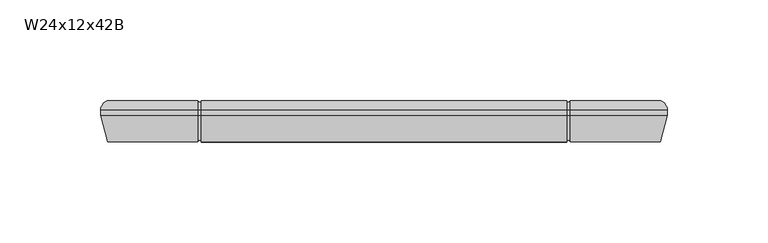
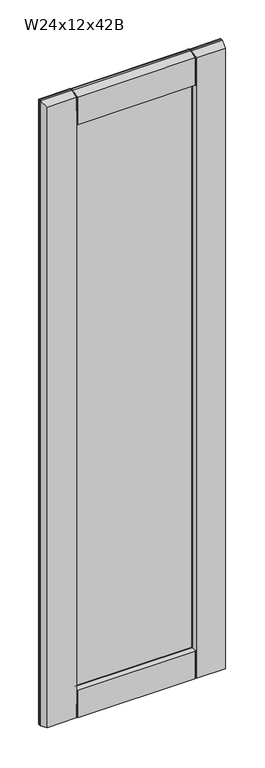
"""IFC4 building model written with IfcOpenShell, lengths in millimetres: furniture geometry, Cabinet-Wall-Merillat-Double_Door-Marlin : W24x12x42B."""

from ifc_helpers import new_model, si_unit, frame, origin, place, context, project, spatial, polyline, circle_curve, ellipse_curve, outline, extrude, source, transform, mapped, element, save
from ifc_brep_helpers import plane_surface, cylinder_surface, advanced_brep


def w24x12x42b_e979b61e(model_context):
    return source(origin(), model_context, "Body", "SolidModel", [
        advanced_brep(
        [(541.0528392, 382.5621, 2108.2), (541.0528392, 382.5621, 1092.2), (537.9563467, 387.0325, 1095.2964925), (537.9563467, 387.0325, 2105.1035075), (541.0528392, 379.7935, 2108.2), (541.0528392, 379.7935, 1092.2), (537.5476392, 366.7125, 2104.6948), (537.5476392, 366.7125, 1095.7052), (492.8516765, 366.7125, 2059.9988372), (492.4815448, 367.50625, 2059.6287055), (490.4003857, 371.96931, 2057.5475465), (490.4003857, 371.96931, 1142.8524535), (492.4815448, 367.50625, 1140.7712945), (492.8516765, 366.7125, 1140.4011628), (491.8001552, 374.2094093, 2058.947316), (491.8001552, 374.2094093, 1141.452684), (506.1278392, 374.4595, 2073.275), (506.1278392, 374.4595, 1127.125), (506.1278392, 379.2855, 2073.275), (506.1278392, 379.2855, 1127.125), (491.8001552, 379.5355907, 2058.947316), (491.8001552, 379.5355907, 1141.452684), (490.4003857, 381.77569, 2057.5475465), (490.4003857, 381.77569, 1142.8524535), (492.4815448, 386.23875, 2059.6287055), (492.848809, 387.0263508, 2059.9959698), (492.8516765, 387.0325, 1140.4011628), (492.4815448, 386.23875, 1140.7712945), (263.1618317, 387.0325, 1095.2964925), (308.2295579, 387.0325, 1095.2964925), (308.2295579, 382.5621, 1092.2), (260.0653392, 382.5621, 1092.2), (492.848809, 382.5621, 1092.2), (492.848809, 387.0325, 1095.2964925), (491.261309, 382.5621, 1092.2), (309.8170579, 382.5621, 1092.2), (309.8170579, 387.0325, 1095.2964925), (491.261309, 387.0325, 1095.2964925), (308.2295579, 379.7935, 1092.2), (260.0653392, 379.7935, 1092.2), (492.848809, 379.7935, 1092.2), (491.261309, 379.7935, 1092.2), (309.8170579, 379.7935, 1092.2), (308.2295579, 366.7125, 1095.7052), (263.5705392, 366.7125, 1095.7052), (491.261309, 366.7125, 1095.7052), (309.8170579, 366.7125, 1095.7052), (492.848809, 366.7125, 1095.7052), (310.7177927, 371.96931, 1142.8524535), (308.6366337, 367.50625, 1140.7712945), (309.8170579, 367.50625, 1140.7712945), (309.8170579, 366.7125, 1140.4011628), (491.261309, 366.7125, 1140.4011628), (491.261309, 367.50625, 1140.7712945), (309.3180233, 374.2094093, 1141.452684), (294.9903392, 374.4595, 1127.125), (294.9903392, 379.2855, 1127.125), (309.3180233, 379.5355907, 1141.452684), (310.7177927, 381.77569, 1142.8524535), (491.261309, 386.23875, 1140.7712945), (491.261309, 387.0325, 1140.4011628), (309.8170579, 387.0325, 1140.4011628), (309.8170579, 386.23875, 1140.7712945), (308.6366337, 386.23875, 1140.7712945), (260.0653392, 382.5621, 2108.2), (263.1618317, 387.0325, 2105.1035075), (260.0653392, 379.7935, 2108.2), (263.5705392, 366.7125, 2104.6948), (308.266502, 366.7125, 1140.4011628), (310.7177927, 371.96931, 2057.5475465), (308.6366337, 367.50625, 2059.6287055), (308.266502, 366.7125, 2059.9988372), (309.3180233, 374.2094093, 2058.947316), (294.9903392, 374.4595, 2073.275), (294.9903392, 379.2855, 2073.275), (309.3180233, 379.5355907, 2058.947316), (310.7177927, 381.77569, 2057.5475465), (308.266502, 387.0325, 1140.4011628), (308.266502, 387.0325, 2059.9988372), (308.6366337, 386.23875, 2059.6287055), (492.848809, 387.0325, 2105.1035075), (492.848809, 382.5621, 2108.2), (308.2295579, 382.5621, 2108.2), (308.2295579, 387.0325, 2105.1035075), (309.8170579, 382.5621, 2108.2), (491.261309, 382.5621, 2108.2), (491.261309, 387.0325, 2105.1035075), (309.8170579, 387.0325, 2105.1035075), (492.848809, 379.7935, 2108.2), (308.2295579, 379.7935, 2108.2), (309.8170579, 379.7935, 2108.2), (491.261309, 379.7935, 2108.2), (492.848809, 366.7125, 2104.6948), (308.2295579, 366.7125, 2104.6948), (309.8170579, 366.7125, 2104.6948), (491.261309, 366.7125, 2104.6948), (309.8170579, 366.7125, 2059.9988372), (491.261309, 366.7125, 2059.9988372), (491.261309, 367.50625, 2059.6287055), (309.8170579, 367.50625, 2059.6287055), (309.8170579, 386.23875, 2059.6287055), (309.8170579, 387.0325, 2059.9988372), (491.261309, 387.0325, 2059.9988372), (491.261309, 386.23875, 2059.6287055), (309.8170579, 386.23875, 2104.9526052), (309.8170579, 382.5621, 2107.40625), (309.8170579, 379.8980037, 2107.40625), (309.8170579, 367.50625, 2104.0857412), (308.2295579, 367.50625, 2059.6287055), (308.2295579, 367.50625, 2104.0857412), (308.2295579, 379.8980037, 2107.40625), (308.2295579, 382.5621, 2107.40625), (308.2295579, 386.23875, 2104.9526052), (308.2295579, 386.23875, 2059.6287055), (492.848809, 386.23875, 2059.6287055), (492.848809, 386.23875, 2104.9526052), (492.848809, 382.5621, 2107.40625), (492.848809, 379.8980037, 2107.40625), (492.848809, 367.50625, 2104.0857412), (492.848809, 367.50625, 2059.6287055), (491.261309, 367.50625, 2104.0857412), (491.261309, 379.8980037, 2107.40625), (491.261309, 382.5621, 2107.40625), (491.261309, 386.23875, 2104.9526052), (492.848809, 367.50625, 1140.7712945), (492.848809, 367.50625, 1096.3142588), (492.848809, 379.8980037, 1092.99375), (492.848809, 382.5621, 1092.99375), (492.848809, 386.23875, 1095.4473948), (492.848809, 386.23875, 1140.7712945), (491.261309, 386.23875, 1095.4473948), (491.261309, 382.5621, 1092.99375), (491.261309, 379.8980037, 1092.99375), (491.261309, 367.50625, 1096.3142588), (309.8170579, 367.50625, 1096.3142588), (309.8170579, 379.8980037, 1092.99375), (309.8170579, 382.5621, 1092.99375), (309.8170579, 386.23875, 1095.4473948), (308.2295579, 386.23875, 1140.7712945), (308.2295579, 386.23875, 1095.4473948), (308.2295579, 382.5621, 1092.99375), (308.2295579, 379.8980037, 1092.99375), (308.2295579, 367.50625, 1096.3142588), (308.2295579, 367.50625, 1140.7712945)],
        [
            (0, 1),
            (1, 2, ellipse_curve(frame((536.2776392, 382.5621, 1096.9752), z_axis=(0.7071067811865475, 0.0, 0.7071067811865475), x_axis=(-0.7071067811865474, 0.0, 0.7071067811865476)), 6.7531526, 4.7752)),
            (2, 3),
            (3, 0, ellipse_curve(frame((536.2776392, 382.5621, 2103.4248), z_axis=(0.7071067811865475, 0.0, -0.7071067811865475), x_axis=(0.7071067811865474, 0.0, 0.7071067811865476)), 6.7531526, 4.7752)),
            (0, 4),
            (4, 5),
            (5, 1),
            (4, 6),
            (6, 7),
            (7, 5),
            (8, 9),
            (9, 10),
            (10, 11),
            (11, 12),
            (12, 13),
            (13, 8),
            (10, 14, ellipse_curve(frame((491.8276392, 372.6348492, 2058.9748), z_axis=(0.7071067811865475, 0.0, -0.7071067811865475), x_axis=(0.7071067811865474, 0.0, 0.7071067811865476)), 2.2271035, 1.5748)),
            (14, 15),
            (15, 11, ellipse_curve(frame((491.8276392, 372.6348492, 1141.4252), z_axis=(0.7071067811865475, 0.0, 0.7071067811865475), x_axis=(-0.7071067811865474, 0.0, 0.7071067811865476)), 2.2271035, 1.5748)),
            (14, 16),
            (16, 17),
            (17, 15),
            (16, 18),
            (18, 19),
            (19, 17),
            (18, 20),
            (20, 21),
            (21, 19),
            (20, 22, ellipse_curve(frame((491.8276392, 381.1101508, 2058.9748), z_axis=(0.7071067811865475, 0.0, -0.7071067811865475), x_axis=(0.7071067811865474, 0.0, 0.7071067811865476)), 2.2271035, 1.5748)),
            (22, 23),
            (23, 21, ellipse_curve(frame((491.8276392, 381.1101508, 1141.4252), z_axis=(0.7071067811865475, 0.0, 0.7071067811865475), x_axis=(-0.7071067811865474, 0.0, 0.7071067811865476)), 2.2271035, 1.5748)),
            (22, 24),
            (24, 25),
            (25, 26),
            (26, 27),
            (27, 23),
            (28, 29),
            (29, 30, circle_curve(frame((308.2295579, 382.5621, 1096.9752), z_axis=(-1.0, 0.0, 0.0), x_axis=(0.0, -1.0, 0.0)), 4.7752)),
            (30, 31),
            (31, 28, ellipse_curve(frame((264.8405392, 382.5621, 1096.9752), z_axis=(0.7071067811865475, 0.0, -0.7071067811865475), x_axis=(0.7071067811865476, 0.0, 0.7071067811865474)), 6.7531526, 4.7752)),
            (1, 32),
            (32, 33, circle_curve(frame((492.848809, 382.5621, 1096.9752), z_axis=(1.0, 0.0, 0.0), x_axis=(0.0, -1.0, 0.0)), 4.7752)),
            (33, 2),
            (34, 35),
            (35, 36, circle_curve(frame((309.8170579, 382.5621, 1096.9752), z_axis=(1.0, 0.0, 0.0), x_axis=(0.0, -1.0, 0.0)), 4.7752)),
            (36, 37),
            (37, 34, circle_curve(frame((491.261309, 382.5621, 1096.9752), z_axis=(-1.0, 0.0, 0.0), x_axis=(0.0, -1.0, 0.0)), 4.7752)),
            (30, 38),
            (38, 39),
            (39, 31),
            (5, 40),
            (40, 32),
            (41, 42),
            (42, 35),
            (34, 41),
            (38, 43),
            (43, 44),
            (44, 39),
            (45, 46),
            (46, 42),
            (41, 45),
            (7, 47),
            (47, 40),
            (48, 49),
            (49, 50),
            (50, 51),
            (51, 52),
            (52, 53),
            (53, 12),
            (11, 48),
            (15, 54),
            (54, 48, ellipse_curve(frame((309.2905392, 372.6348492, 1141.4252), z_axis=(0.7071067811865475, 0.0, -0.7071067811865475), x_axis=(0.7071067811865476, 0.0, 0.7071067811865474)), 2.2271035, 1.5748)),
            (17, 55),
            (55, 54),
            (19, 56),
            (56, 55),
            (21, 57),
            (57, 56),
            (23, 58),
            (58, 57, ellipse_curve(frame((309.2905392, 381.1101508, 1141.4252), z_axis=(0.7071067811865475, 0.0, -0.7071067811865475), x_axis=(0.7071067811865476, 0.0, 0.7071067811865474)), 2.2271035, 1.5748)),
            (27, 59),
            (59, 60),
            (60, 61),
            (61, 62),
            (62, 63),
            (63, 58),
            (31, 64),
            (64, 65, ellipse_curve(frame((264.8405392, 382.5621, 2103.4248), z_axis=(-0.7071067811865475, 0.0, -0.7071067811865475), x_axis=(0.7071067811865474, 0.0, -0.7071067811865476)), 6.7531526, 4.7752)),
            (65, 28),
            (39, 66),
            (66, 64),
            (44, 67),
            (67, 66),
            (68, 49),
            (48, 69),
            (69, 70),
            (70, 71),
            (71, 68),
            (54, 72),
            (72, 69, ellipse_curve(frame((309.2905392, 372.6348492, 2058.9748), z_axis=(-0.7071067811865475, 0.0, -0.7071067811865475), x_axis=(0.7071067811865474, 0.0, -0.7071067811865476)), 2.2271035, 1.5748)),
            (55, 73),
            (73, 72),
            (56, 74),
            (74, 73),
            (57, 75),
            (75, 74),
            (58, 76),
            (76, 75, ellipse_curve(frame((309.2905392, 381.1101508, 2058.9748), z_axis=(-0.7071067811865475, 0.0, -0.7071067811865475), x_axis=(0.7071067811865474, 0.0, -0.7071067811865476)), 2.2271035, 1.5748)),
            (63, 77),
            (77, 78),
            (78, 79),
            (79, 76),
            (3, 80),
            (80, 81, circle_curve(frame((492.848809, 382.5621, 2103.4248), z_axis=(1.0, 0.0, 0.0), x_axis=(0.0, -1.0, 0.0)), 4.7752)),
            (81, 0),
            (64, 82),
            (82, 83, circle_curve(frame((308.2295579, 382.5621, 2103.4248), z_axis=(-1.0, 0.0, 0.0), x_axis=(0.0, -1.0, 0.0)), 4.7752)),
            (83, 65),
            (84, 85),
            (85, 86, circle_curve(frame((491.261309, 382.5621, 2103.4248), z_axis=(-1.0, 0.0, 0.0), x_axis=(0.0, -1.0, 0.0)), 4.7752)),
            (86, 87),
            (87, 84, circle_curve(frame((309.8170579, 382.5621, 2103.4248), z_axis=(1.0, 0.0, 0.0), x_axis=(0.0, -1.0, 0.0)), 4.7752)),
            (81, 88),
            (88, 4),
            (66, 89),
            (89, 82),
            (90, 91),
            (91, 85),
            (84, 90),
            (88, 92),
            (92, 6),
            (67, 93),
            (93, 89),
            (94, 95),
            (95, 91),
            (90, 94),
            (51, 46),
            (45, 52),
            (43, 68),
            (71, 93),
            (92, 8),
            (13, 47),
            (96, 97),
            (97, 95),
            (94, 96),
            (9, 98),
            (98, 97),
            (96, 99),
            (99, 70),
            (69, 10),
            (72, 14),
            (73, 16),
            (74, 18),
            (75, 20),
            (76, 22),
            (79, 100),
            (100, 101),
            (101, 102),
            (102, 103),
            (103, 24),
            (33, 26),
            (25, 80),
            (36, 61),
            (60, 37),
            (83, 78),
            (77, 29),
            (86, 102),
            (101, 87),
            (100, 104),
            (104, 105, circle_curve(frame((309.8170579, 382.5621, 2103.4248), z_axis=(1.0, 0.0, 0.0), x_axis=(0.0, 0.0, 1.0)), 3.98145)),
            (105, 106),
            (106, 107),
            (107, 99),
            (71, 108),
            (108, 109),
            (109, 110),
            (110, 111),
            (111, 112, circle_curve(frame((308.2295579, 382.5621, 2103.4248), z_axis=(-1.0, 0.0, 0.0), x_axis=(0.0, 0.0, 1.0)), 3.98145)),
            (112, 113),
            (113, 78),
            (113, 79),
            (112, 104),
            (111, 105),
            (110, 106),
            (109, 107),
            (108, 70),
            (25, 114),
            (114, 115),
            (115, 116, circle_curve(frame((492.848809, 382.5621, 2103.4248), z_axis=(1.0, 0.0, 0.0), x_axis=(0.0, 0.0, 1.0)), 3.98145)),
            (116, 117),
            (117, 118),
            (118, 119),
            (119, 8),
            (98, 120),
            (120, 121),
            (121, 122),
            (122, 123, circle_curve(frame((491.261309, 382.5621, 2103.4248), z_axis=(-1.0, 0.0, 0.0), x_axis=(0.0, 0.0, 1.0)), 3.98145)),
            (123, 103),
            (24, 114),
            (123, 115),
            (122, 116),
            (121, 117),
            (120, 118),
            (9, 119),
            (13, 124),
            (124, 125),
            (125, 126),
            (126, 127),
            (127, 128, circle_curve(frame((492.848809, 382.5621, 1096.9752), z_axis=(1.0, 0.0, 0.0), x_axis=(0.0, 0.0, 1.0)), 3.98145)),
            (128, 129),
            (129, 26),
            (59, 130),
            (130, 131, circle_curve(frame((491.261309, 382.5621, 1096.9752), z_axis=(-1.0, 0.0, 0.0), x_axis=(0.0, 0.0, 1.0)), 3.98145)),
            (131, 132),
            (132, 133),
            (133, 53),
            (12, 124),
            (133, 125),
            (132, 126),
            (131, 127),
            (130, 128),
            (27, 129),
            (50, 134),
            (134, 135),
            (135, 136),
            (136, 137, circle_curve(frame((309.8170579, 382.5621, 1096.9752), z_axis=(1.0, 0.0, 0.0), x_axis=(0.0, 0.0, 1.0)), 3.98145)),
            (137, 62),
            (138, 139),
            (139, 140, circle_curve(frame((308.2295579, 382.5621, 1096.9752), z_axis=(-1.0, 0.0, 0.0), x_axis=(0.0, 0.0, 1.0)), 3.98145)),
            (140, 141),
            (141, 142),
            (142, 143),
            (143, 68),
            (77, 138),
            (63, 138),
            (143, 49),
            (142, 134),
            (141, 135),
            (140, 136),
            (139, 137),
        ],
        [
            cylinder_surface(frame((536.2776392, 382.5621, 2108.2), z_axis=(0.0, 0.0, 1.0), x_axis=(0.0, -1.0, 0.0)), 4.7752),
            plane_surface(frame((541.0528392, 382.5621, 2108.2), z_axis=(1.0, 0.0, 0.0), x_axis=(0.0, 0.0, -1.0))),
            plane_surface(frame((541.0528392, 379.7935, 2108.2), z_axis=(0.9659229350723619, -0.25882983502910506, 0.0), x_axis=(0.0, 0.0, -1.0))),
            plane_surface(frame((492.8516765, 366.7125, 2059.9988372), z_axis=(-0.9063077870366099, -0.4226182617407856, 0.0), x_axis=(0.0, 0.0, -1.0))),
            cylinder_surface(frame((491.8276392, 372.6348492, 2108.2), z_axis=(0.0, 0.0, 1.0000000000000002), x_axis=(-0.01745240643729364, 0.9998476951563912, 0.0)), 1.5748),
            plane_surface(frame((491.8001552, 374.2094093, 2058.947316), z_axis=(-0.017452406437322144, 0.9998476951563906, 0.0), x_axis=(0.0, 0.0, -1.0))),
            plane_surface(frame((506.1278392, 374.4595, 2073.275), z_axis=(-1.0, 0.0, 0.0), x_axis=(0.0, 0.0, -1.0))),
            plane_surface(frame((506.1278392, 379.2855, 2073.275), z_axis=(-0.01745240643727848, -0.9998476951563914, 0.0), x_axis=(0.0, 0.0, -1.0))),
            cylinder_surface(frame((491.8276392, 381.1101508, 2108.2), z_axis=(0.0, 0.0, 1.0000000000000002), x_axis=(-0.9063077870367326, 0.42261826174052236, 0.0)), 1.5748),
            plane_surface(frame((490.4003857, 381.77569, 2057.5475465), z_axis=(-0.9063077870366333, 0.4226182617407352, 0.0), x_axis=(0.0, 0.0, -1.0))),
            cylinder_surface(frame((541.0528392, 382.5621, 1096.9752), z_axis=(1.0, 0.0, 0.0), x_axis=(0.0, -1.0, 0.0)), 4.7752),
            plane_surface(frame((541.0528392, 382.5621, 1092.2), z_axis=(0.0, 0.0, -1.0), x_axis=(-1.0, 0.0, 0.0))),
            plane_surface(frame((541.0528392, 379.7935, 1092.2), z_axis=(0.0, -0.2588298350291095, -0.9659229350723607), x_axis=(-1.0, 0.0, 0.0))),
            plane_surface(frame((492.8516765, 366.7125, 1140.4011628), z_axis=(0.0, -0.42261826174078143, 0.9063077870366119), x_axis=(-1.0, 0.0, 0.0))),
            cylinder_surface(frame((541.0528392, 372.6348492, 1141.4252), z_axis=(1.0000000000000002, 0.0, 0.0), x_axis=(0.0, 0.9998476951563913, 0.017452406437289025)), 1.5748),
            plane_surface(frame((491.8001552, 374.2094093, 1141.452684), z_axis=(0.0, 0.9998476951563907, 0.01745240643731753), x_axis=(-1.0, 0.0, 0.0))),
            plane_surface(frame((506.1278392, 374.4595, 1127.125), z_axis=(0.0, 0.0, 1.0), x_axis=(-1.0, 0.0, 0.0))),
            plane_surface(frame((506.1278392, 379.2855, 1127.125), z_axis=(0.0, -0.9998476951563913, 0.017452406437283095), x_axis=(-1.0, 0.0, 0.0))),
            cylinder_surface(frame((541.0528392, 381.1101508, 1141.4252), z_axis=(1.0000000000000002, 0.0, 0.0), x_axis=(0.0, 0.4226182617405265, 0.9063077870367306)), 1.5748),
            plane_surface(frame((490.4003857, 381.77569, 1142.8524535), z_axis=(0.0, 0.4226182617407394, 0.9063077870366314), x_axis=(-1.0, 0.0, 0.0))),
            cylinder_surface(frame((264.8405392, 382.5621, 1092.2), z_axis=(0.0, 0.0, -1.0), x_axis=(0.0, -1.0, 0.0)), 4.7752),
            plane_surface(frame((260.0653392, 382.5621, 1092.2), z_axis=(-1.0, 0.0, 0.0), x_axis=(0.0, 0.0, 1.0))),
            plane_surface(frame((260.0653392, 379.7935, 1092.2), z_axis=(-0.9659229350723619, -0.25882983502910506, 0.0), x_axis=(0.0, 0.0, 1.0))),
            plane_surface(frame((308.266502, 366.7125, 1140.4011628), z_axis=(0.9063077870366099, -0.4226182617407856, 0.0), x_axis=(0.0, 0.0, 1.0))),
            cylinder_surface(frame((309.2905392, 372.6348492, 1092.2), z_axis=(0.0, 0.0, -1.0000000000000002), x_axis=(0.01745240643729364, 0.9998476951563912, 0.0)), 1.5748),
            plane_surface(frame((309.3180233, 374.2094093, 1141.452684), z_axis=(0.017452406437322144, 0.9998476951563906, 0.0), x_axis=(0.0, 0.0, 1.0))),
            plane_surface(frame((294.9903392, 374.4595, 1127.125), z_axis=(1.0, 0.0, 0.0), x_axis=(0.0, 0.0, 1.0))),
            plane_surface(frame((294.9903392, 379.2855, 1127.125), z_axis=(0.01745240643727848, -0.9998476951563914, 0.0), x_axis=(0.0, 0.0, 1.0))),
            cylinder_surface(frame((309.2905392, 381.1101508, 1092.2), z_axis=(0.0, 0.0, -1.0000000000000002), x_axis=(0.9063077870367326, 0.42261826174052236, 0.0)), 1.5748),
            plane_surface(frame((310.7177927, 381.77569, 1142.8524535), z_axis=(0.9063077870366333, 0.4226182617407352, 0.0), x_axis=(0.0, 0.0, 1.0))),
            cylinder_surface(frame((260.0653392, 382.5621, 2103.4248), z_axis=(-1.0, 0.0, 0.0), x_axis=(0.0, -1.0, 0.0)), 4.7752),
            plane_surface(frame((260.0653392, 382.5621, 2108.2), z_axis=(0.0, 0.0, 1.0), x_axis=(1.0, 0.0, 0.0))),
            plane_surface(frame((260.0653392, 379.7935, 2108.2), z_axis=(0.0, -0.2588298350291006, 0.9659229350723632), x_axis=(1.0, 0.0, 0.0))),
            plane_surface(frame((263.5705392, 366.7125, 2104.6948), z_axis=(0.0, -1.0, 0.0), x_axis=(1.0, 0.0, 0.0))),
            plane_surface(frame((308.266502, 366.7125, 2059.9988372), z_axis=(0.0, -0.42261826174078976, -0.9063077870366079), x_axis=(1.0, 0.0, 0.0))),
            cylinder_surface(frame((260.0653392, 372.6348492, 2058.9748), z_axis=(-1.0000000000000002, 0.0, 0.0), x_axis=(0.0, 0.999847695156391, -0.017452406437298253)), 1.5748),
            plane_surface(frame((309.3180233, 374.2094093, 2058.947316), z_axis=(0.0, 0.9998476951563905, -0.01745240643732676), x_axis=(1.0, 0.0, 0.0))),
            plane_surface(frame((294.9903392, 374.4595, 2073.275), z_axis=(0.0, 0.0, -1.0), x_axis=(1.0, 0.0, 0.0))),
            plane_surface(frame((294.9903392, 379.2855, 2073.275), z_axis=(0.0, -0.9998476951563915, -0.017452406437273867), x_axis=(1.0, 0.0, 0.0))),
            cylinder_surface(frame((260.0653392, 381.1101508, 2058.9748), z_axis=(-1.0000000000000002, 0.0, 0.0), x_axis=(0.0, 0.4226182617405182, -0.9063077870367346)), 1.5748),
            plane_surface(frame((310.7177927, 381.77569, 2057.5475465), z_axis=(0.0, 0.422618261740731, -0.9063077870366353), x_axis=(1.0, 0.0, 0.0))),
            plane_surface(frame((308.266502, 387.0325, 2059.9988372), z_axis=(0.0, 1.0, 0.0), x_axis=(1.0, 0.0, 0.0))),
            plane_surface(frame((309.8170579, 387.0325, 2059.9988372), z_axis=(-1.0, 0.0, 0.0), x_axis=(0.0, -0.9063077870366119, -0.4226182617407812))),
            plane_surface(frame((308.2295579, 387.0325, 2059.9988372), z_axis=(1.0, 0.0, 0.0), x_axis=(0.0, 0.9063077870366119, 0.4226182617407812))),
            plane_surface(frame((309.8170579, 387.0325, 2059.9988372), z_axis=(0.0, -0.4226182617407812, 0.9063077870366119), x_axis=(-1.0, 0.0, 0.0))),
            plane_surface(frame((309.8170579, 386.23875, 2059.6287055), z_axis=(0.0, 1.0, 0.0), x_axis=(-1.0, 0.0, 0.0))),
            cylinder_surface(frame((308.2295579, 382.5621, 2103.4248), z_axis=(-1.0, 0.0, 0.0), x_axis=(0.0, 0.0, 1.0)), 3.98145),
            plane_surface(frame((309.8170579, 382.5621, 2107.40625), z_axis=(0.0, 0.0, 1.0), x_axis=(-1.0, 0.0, 0.0))),
            plane_surface(frame((309.8170579, 379.8980037, 2107.40625), z_axis=(0.0, -0.25882983502916007, 0.9659229350723473), x_axis=(-1.0, 0.0, 0.0))),
            plane_surface(frame((309.8170579, 367.50625, 2104.0857412), z_axis=(0.0, -1.0, 0.0), x_axis=(-1.0, 0.0, 0.0))),
            plane_surface(frame((309.8170579, 367.50625, 2059.6287055), z_axis=(0.0, 0.4226182617408151, 0.906307787036596), x_axis=(-1.0, 0.0, 0.0))),
            plane_surface(frame((492.848809, 387.0325, 2059.9988372), z_axis=(-1.0, 0.0, 0.0), x_axis=(0.0, -0.9063077870366119, -0.4226182617407812))),
            plane_surface(frame((491.261309, 387.0325, 2059.9988372), z_axis=(1.0, 0.0, 0.0), x_axis=(0.0, 0.9063077870366119, 0.4226182617407812))),
            plane_surface(frame((492.848809, 387.0325, 2059.9988372), z_axis=(0.0, -0.4226182617407812, 0.9063077870366119), x_axis=(-1.0, 0.0, 0.0))),
            plane_surface(frame((492.848809, 386.23875, 2059.6287055), z_axis=(0.0, 1.0, 0.0), x_axis=(-1.0, 0.0, 0.0))),
            cylinder_surface(frame((491.261309, 382.5621, 2103.4248), z_axis=(-1.0, 0.0, 0.0), x_axis=(0.0, 0.0, 1.0)), 3.98145),
            plane_surface(frame((492.848809, 382.5621, 2107.40625), z_axis=(0.0, 0.0, 1.0), x_axis=(-1.0, 0.0, 0.0))),
            plane_surface(frame((492.848809, 379.8980037, 2107.40625), z_axis=(0.0, -0.25882983502916257, 0.9659229350723466), x_axis=(-1.0, 0.0, 0.0))),
            plane_surface(frame((492.848809, 367.50625, 2104.0857412), z_axis=(0.0, -1.0, 0.0), x_axis=(-1.0, 0.0, 0.0))),
            plane_surface(frame((492.848809, 367.50625, 2059.6287055), z_axis=(0.0, 0.42261826174081607, 0.9063077870365956), x_axis=(-1.0, 0.0, 0.0))),
            plane_surface(frame((492.848809, 382.5621, 1101.7504), z_axis=(-1.0, 0.0, 0.0), x_axis=(0.0, 1.0, 0.0))),
            plane_surface(frame((491.261309, 382.5621, 1101.7504), z_axis=(1.0, 0.0, 0.0), x_axis=(0.0, -1.0, 0.0))),
            plane_surface(frame((492.848809, 366.7125, 1140.4011628), z_axis=(0.0, 0.4226182617407898, -0.906307787036608), x_axis=(-1.0, 0.0, 0.0))),
            plane_surface(frame((492.848809, 367.50625, 1140.7712945), z_axis=(0.0, -1.0, 0.0), x_axis=(-1.0, 0.0, 0.0))),
            plane_surface(frame((492.848809, 367.50625, 1096.3142588), z_axis=(0.0, -0.2588298350294553, -0.9659229350722681), x_axis=(-1.0, 0.0, 0.0))),
            plane_surface(frame((492.848809, 379.8980037, 1092.99375), z_axis=(0.0, 0.0, -1.0), x_axis=(-1.0, 0.0, 0.0))),
            cylinder_surface(frame((491.261309, 382.5621, 1096.9752), z_axis=(-1.0, 0.0, 0.0), x_axis=(0.0, 0.0, 1.0)), 3.98145),
            plane_surface(frame((492.848809, 386.23875, 1095.4473948), z_axis=(0.0, 1.0, 0.0), x_axis=(-1.0, 0.0, 0.0))),
            plane_surface(frame((492.848809, 386.23875, 1140.7712945), z_axis=(0.0, -0.42261826174079614, -0.9063077870366049), x_axis=(-1.0, 0.0, 0.0))),
            plane_surface(frame((309.8170579, 386.23875, 1140.7712945), z_axis=(-1.0000000000000002, 0.0, 0.0), x_axis=(0.0, 0.9063077870366271, -0.4226182617407486))),
            plane_surface(frame((308.2295579, 386.23875, 1140.7712945), z_axis=(1.0000000000000002, 0.0, 0.0), x_axis=(0.0, -0.9063077870366271, 0.4226182617407486))),
            plane_surface(frame((309.8170579, 386.23875, 1140.7712945), z_axis=(0.0, -0.4226182617407486, -0.9063077870366271), x_axis=(-1.0, 0.0, 0.0))),
            plane_surface(frame((309.8170579, 366.7125, 1140.4011628), z_axis=(0.0, 0.4226182617407898, -0.906307787036608), x_axis=(-1.0, 0.0, 0.0))),
            plane_surface(frame((309.8170579, 367.50625, 1140.7712945), z_axis=(0.0, -1.0, 0.0), x_axis=(-1.0, 0.0, 0.0))),
            plane_surface(frame((309.8170579, 367.50625, 1096.3142588), z_axis=(0.0, -0.25882983502945534, -0.9659229350722681), x_axis=(-1.0, 0.0, 0.0))),
            plane_surface(frame((309.8170579, 379.8980037, 1092.99375), z_axis=(0.0, 0.0, -1.0), x_axis=(-1.0, 0.0, 0.0))),
            cylinder_surface(frame((308.2295579, 382.5621, 1096.9752), z_axis=(-1.0, 0.0, 0.0), x_axis=(0.0, 0.0, 1.0)), 3.98145),
            plane_surface(frame((309.8170579, 386.23875, 1095.4473948), z_axis=(0.0, 1.0, 0.0), x_axis=(-1.0, 0.0, 0.0))),
        ],
        [
            (0, [[1, 2, 3, 4]]),
            (1, [[5, 6, 7, -1]]),
            (2, [[8, 9, 10, -6]]),
            (3, [[11, 12, 13, 14, 15, 16]]),
            (4, [[17, 18, 19, -13]]),
            (5, [[20, 21, 22, -18]]),
            (6, [[23, 24, 25, -21]]),
            (7, [[26, 27, 28, -24]]),
            (8, [[29, 30, 31, -27]]),
            (9, [[32, 33, 34, 35, 36, -30]]),
            (10, [[37, 38, 39, 40]]),
            (10, [[41, 42, 43, -2]]),
            (10, [[44, 45, 46, 47]]),
            (11, [[-39, 48, 49, 50]]),
            (11, [[51, 52, -41, -7]]),
            (11, [[53, 54, -44, 55]]),
            (12, [[-49, 56, 57, 58]]),
            (12, [[59, 60, -53, 61]]),
            (12, [[62, 63, -51, -10]]),
            (13, [[64, 65, 66, 67, 68, 69, -14, 70]]),
            (14, [[71, 72, -70, -19]]),
            (15, [[73, 74, -71, -22]]),
            (16, [[75, 76, -73, -25]]),
            (17, [[77, 78, -75, -28]]),
            (18, [[79, 80, -77, -31]]),
            (19, [[-36, 81, 82, 83, 84, 85, 86, -79]]),
            (20, [[87, 88, 89, -40]]),
            (21, [[90, 91, -87, -50]]),
            (22, [[92, 93, -90, -58]]),
            (23, [[94, -64, 95, 96, 97, 98]]),
            (24, [[99, 100, -95, -72]]),
            (25, [[101, 102, -99, -74]]),
            (26, [[103, 104, -101, -76]]),
            (27, [[105, 106, -103, -78]]),
            (28, [[107, 108, -105, -80]]),
            (29, [[-86, 109, 110, 111, 112, -107]]),
            (30, [[113, 114, 115, -4]]),
            (30, [[116, 117, 118, -88]]),
            (30, [[119, 120, 121, 122]]),
            (31, [[-115, 123, 124, -5]]),
            (31, [[125, 126, -116, -91]]),
            (31, [[127, 128, -119, 129]]),
            (32, [[-124, 130, 131, -8]]),
            (32, [[132, 133, -125, -93]]),
            (32, [[134, 135, -127, 136]]),
            (33, [[-67, 137, -59, 138]]),
            (33, [[-57, 139, -98, 140, -132, -92]]),
            (33, [[-131, 141, -16, 142, -62, -9]]),
            (33, [[143, 144, -134, 145]]),
            (34, [[-12, 146, 147, -143, 148, 149, -96, 150]]),
            (35, [[-150, -100, 151, -17]]),
            (36, [[-151, -102, 152, -20]]),
            (37, [[-152, -104, 153, -23]]),
            (38, [[-153, -106, 154, -26]]),
            (39, [[-154, -108, 155, -29]]),
            (40, [[-112, 156, 157, 158, 159, 160, -32, -155]]),
            (41, [[-43, 161, -34, 162, -113, -3]]),
            (41, [[-46, 163, -83, 164]]),
            (41, [[-118, 165, -110, 166, -37, -89]]),
            (41, [[-121, 167, -158, 168]]),
            (42, [[-148, -145, -136, -129, -122, -168, -157, 169, 170, 171, 172, 173]]),
            (43, [[-165, -117, -126, -133, -140, 174, 175, 176, 177, 178, 179, 180]]),
            (44, [[181, -111, -180]]),
            (45, [[-156, -181, -179, 182, -169]]),
            (46, [[-182, -178, 183, -170]]),
            (47, [[-183, -177, 184, -171]]),
            (48, [[-184, -176, 185, -172]]),
            (49, [[-185, -175, 186, -149, -173]]),
            (50, [[-97, -186, -174]]),
            (51, [[-141, -130, -123, -114, -162, 187, 188, 189, 190, 191, 192, 193]]),
            (52, [[-159, -167, -120, -128, -135, -144, -147, 194, 195, 196, 197, 198]]),
            (53, [[-33, 199, -187]]),
            (54, [[-199, -160, -198, 200, -188]]),
            (55, [[-200, -197, 201, -189]]),
            (56, [[-201, -196, 202, -190]]),
            (57, [[-202, -195, 203, -191]]),
            (58, [[-203, -194, -146, 204, -192]]),
            (59, [[-204, -11, -193]]),
            (60, [[-161, -42, -52, -63, -142, 205, 206, 207, 208, 209, 210, 211]]),
            (61, [[-68, -138, -61, -55, -47, -164, -82, 212, 213, 214, 215, 216]]),
            (62, [[-15, 217, -205]]),
            (63, [[-217, -69, -216, 218, -206]]),
            (64, [[-218, -215, 219, -207]]),
            (65, [[-219, -214, 220, -208]]),
            (66, [[-220, -213, 221, -209]]),
            (67, [[-221, -212, -81, 222, -210]]),
            (68, [[-222, -35, -211]]),
            (69, [[-84, -163, -45, -54, -60, -137, -66, 223, 224, 225, 226, 227]]),
            (70, [[228, 229, 230, 231, 232, 233, -139, -56, -48, -38, -166, 234]]),
            (71, [[-109, 235, -234]]),
            (72, [[236, -94, -233]]),
            (73, [[-65, -236, -232, 237, -223]]),
            (74, [[-237, -231, 238, -224]]),
            (75, [[-238, -230, 239, -225]]),
            (76, [[-239, -229, 240, -226]]),
            (77, [[-240, -228, -235, -85, -227]]),
        ],
    ),
        extrude(outline(polyline([(294.9903392, 379.2855), (506.1278392, 379.2855), (506.1278392, 374.4595), (294.9903392, 374.4595), (294.9903392, 379.2855)])), frame((0.0, 0.0, 1127.125), z_axis=(0.0, 0.0, 1.0), x_axis=(1.0, 0.0, 0.0)), (0.0, 0.0, 1.0), 946.15),
    ])


if __name__ == "__main__":
    model = new_model("IFC4")
    model_context = context("Model", 3, world=origin())
    ifc_project = project(units=[si_unit("LENGTHUNIT", "METRE", prefix="MILLI")], contexts=[model_context])
    site = spatial("IfcSite", under=ifc_project)
    building = spatial("IfcBuilding", under=site)
    placement = place(None, origin())
    w24x12x42b_shape = w24x12x42b_e979b61e(model_context)
    element("IfcFurniture", 1, ObjectType="Cabinet-Wall-Merillat-Double_Door-Marlin : W24x12x42B", at=placement, inside=building, context=model_context, shape_type="MappedRepresentation", body=[
        mapped(w24x12x42b_shape, transform((0.0, 0.0, 0.0), x_axis=(1.0, 0.0, 0.0), y_axis=(0.0, 1.0, 0.0), z_axis=(0.0, 0.0, 1.0))),
    ])
    save(model, "model.ifc")

# Revit data of these elements
# Type "Cabinet-Wall-Merillat-Double_Door-Marlin : W24x12x42B"
#   URL = "https://www.merillat.com/"
#   Product Page URL = "https://www.merillat.com/our-products/"
#   Product Line = "Express"
#   Product Group = "Wall Cabinet"
#   Product Documentation Link = "http://merillatbusiness.com/wp-content/uploads/2014/07/Merillat_Classic_Catalog.pdf"
#   Model = "W2442B"
#   Manufacturer = "Merillat"
#   Height Note = "Actual Height of 21 inches Cabinet is 20 1/2 inches"
#   Glass Door Note = "Glass Cabinet doors are only available in specific sizes. Please refer to the catalog for this information before requesting a glass size."
#   Finish = "Wood"
#   Description = "Wall 2442 Butt Door"
#   Construction Type = "Wall Cabinet"
#   Cabinet Construction Note = "Cabinets with B suffix have BUTT doors without a center frame stile:"
#   Assembly Code = "C1030410"
#   Spacing = 0' - 1"
#   Shelving Height = 0' - 9 3/4"
#   Door Spacing = 0' - 0 1/8"
#   Cabinet Door Width = 0' - 11 1/16"
#   Cabinet Door Height = 3' - 4"
#   Depth = 1' - 0"
#   Height = 3' - 6"
#   Top Of Cabinet = 7' - 0"
#   Width = 2' - 0"
#   COBie.Type = no
#   Top and Bottom Visibility = yes
#   Partial Overlay Butt = yes
#   Partial Overlay = no
#   Number of Shelves Greater than one = 3
#   Number of Shelves = 3
#   Middle Shelf = yes
#   Full Overlay Butt = no
#   Full Overlay = no
#   Elevation Swing Line = yes
#   Door Drawer Material = Wood - Merillat - Pecan(1)
#   Cabinet Material = Wood - Merillat - Pecan(1)
#   Cabinet Door Style = element 806847
# Element 1 (IfcFurniture, "Cabinet-Wall-Merillat-Double_Door-Marlin : W24x12x42B")
#   Materials on its faces: "Wood - Merillat - Pecan(1)"
# Materials
#   "Wood - Merillat - Pecan(1)": class "Wood", colour RGB 108 67 43, transparency 0, Cost = 0
